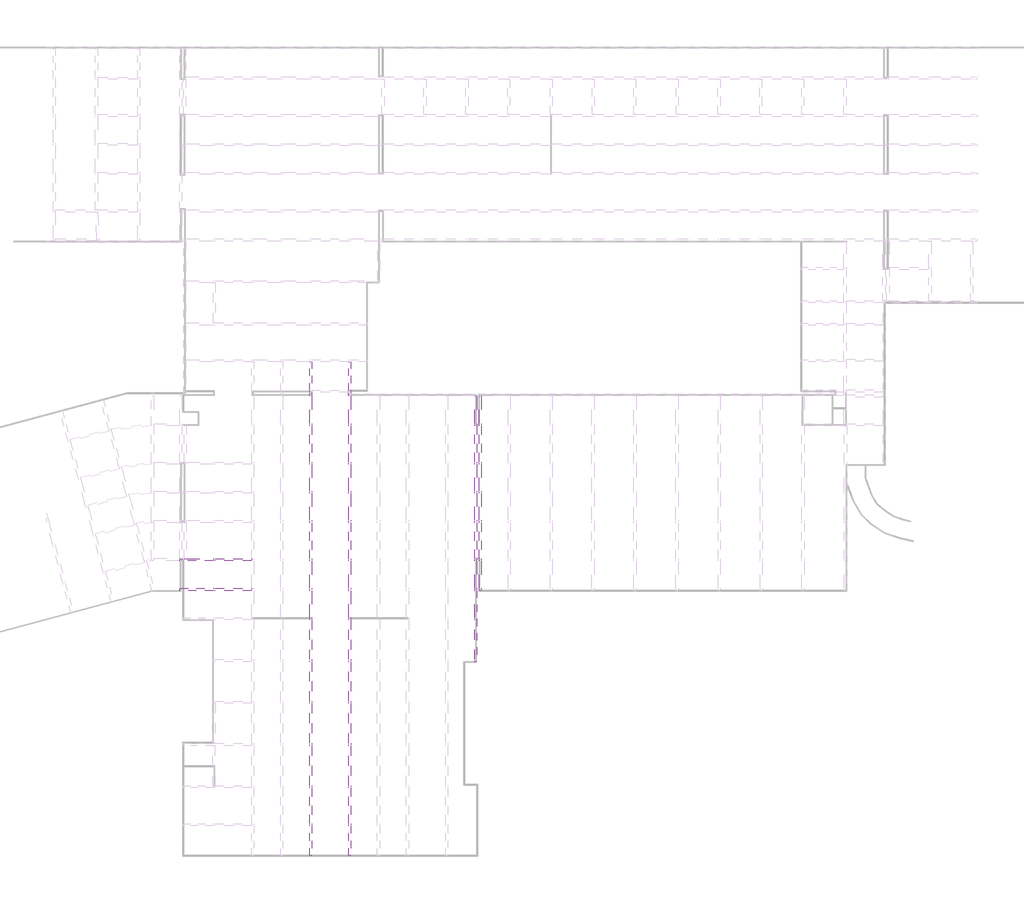
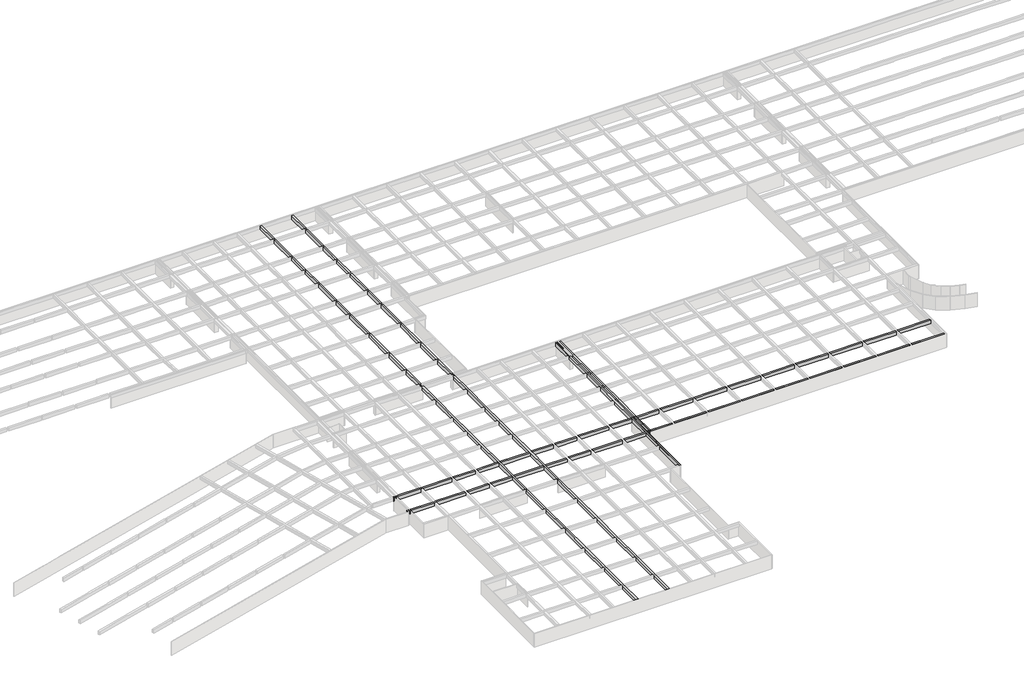
# One storey, part 8 of 14: 6 beams.
"""IFC4 building model written with IfcOpenShell, lengths in millimetres."""

import ifcopenshell
import ifcopenshell.guid

model = None  # the IFC model being written
_history = None  # IfcOwnerHistory: only IFC2X3 demands one
_inside = {}  # id of a spatial element -> (the spatial element, [elements in it])
_under = {}  # id of a project, library or spatial element -> (it, [spatial elements below it])
_declared = {}  # id of a project -> (the project, [libraries it declares])
_typed = {}  # id of a type object -> (the type object, [elements of that type])
_made_of = {}  # id of a material, layer set ... -> (it, [elements and type objects made of it])


def new_model(schema):
    """Start an empty IFC model of exactly this schema.

    Asked for "IFC4X3", IfcOpenShell would pick the latest addendum, in which some entities
    have other attributes; the version numbers below select the first issue.
    IFC2X3 requires an IfcOwnerHistory on every rooted entity: one is made here for all.
    """
    global model, _history
    if schema == "IFC4X3":
        model = ifcopenshell.file(schema_version=(4, 3, 0, 0))
    else:
        model = ifcopenshell.file(schema=schema)
    _inside.clear()
    _under.clear()
    _declared.clear()
    _typed.clear()
    _made_of.clear()
    _history = None
    if model.schema == "IFC2X3":
        org = make("IfcOrganization", Name="unknown")
        user = make(
            "IfcPersonAndOrganization",
            ThePerson=make("IfcPerson", FamilyName="unknown"),
            TheOrganization=org,
        )
        app = make(
            "IfcApplication",
            ApplicationDeveloper=org,
            Version="unknown",
            ApplicationFullName="unknown",
            ApplicationIdentifier="unknown",
        )
        _history = make(
            "IfcOwnerHistory",
            OwningUser=user,
            OwningApplication=app,
            ChangeAction="ADDED",
            CreationDate=0,
        )
    return model


def make(cls, **values):
    """One entity of the class cls with the attributes given. An attribute that is None is left unset."""
    return model.create_entity(
        cls, **{name: value for name, value in values.items() if value is not None}
    )


def rooted(cls, **values):
    """An entity with a GlobalId (a new one), such as an element, a storey or a relation."""
    return make(cls, GlobalId=ifcopenshell.guid.new(), OwnerHistory=_history, **values)


def si_unit(unit_type, name, prefix=None):
    """IfcSIUnit, for example si_unit("LENGTHUNIT", "METRE", prefix="MILLI")."""
    return make("IfcSIUnit", UnitType=unit_type, Prefix=prefix, Name=name)


def assignment(units):
    """IfcUnitAssignment: the units of a project."""
    return None if units is None else make("IfcUnitAssignment", Units=units)


def point(xyz):
    """IfcCartesianPoint."""
    return None if xyz is None else make("IfcCartesianPoint", Coordinates=xyz)


def direction(xyz):
    """IfcDirection."""
    return None if xyz is None else make("IfcDirection", DirectionRatios=xyz)


def frame(location, z_axis=None, x_axis=None):
    """IfcAxis2Placement3D, a coordinate frame: its origin and axes. An axis left out is left unset."""
    return make(
        "IfcAxis2Placement3D",
        Location=point(location),
        Axis=direction(z_axis),
        RefDirection=direction(x_axis),
    )


def origin():
    """The frame at (0, 0, 0) with its axes left unset."""
    return frame((0.0, 0.0, 0.0))


def place(relative_to, where):
    """IfcLocalPlacement: puts the frame where relative to a parent placement (None: the world)."""
    return make(
        "IfcLocalPlacement", PlacementRelTo=relative_to, RelativePlacement=where
    )


def context(
    kind, dimensions, precision=None, world=None, true_north=None, identifier=None
):
    """IfcGeometricRepresentationContext, for example the 3D "Model" context."""
    return make(
        "IfcGeometricRepresentationContext",
        ContextIdentifier=identifier,
        ContextType=kind,
        CoordinateSpaceDimension=dimensions,
        Precision=precision,
        WorldCoordinateSystem=world,
        TrueNorth=true_north,
    )


def project(units=None, contexts=None):
    """IfcProject with its units and contexts."""
    return rooted(
        "IfcProject",
        Name="project",
        RepresentationContexts=contexts,
        UnitsInContext=assignment(units),
    )


def spatial(cls, under=None, at=None, **own):
    """A site, building, storey or space (cls), placed at a placement, below another one or the project."""
    s = rooted(cls, ObjectPlacement=at, **own)
    if under is not None:
        _under.setdefault(under.id(), (under, []))[1].append(s)
    return s


def faces_of(points, faces, orient=None, outer=None):
    """IfcFace entities. A face is a list of loops; a loop is a list of indices into points, from 0.

    orient and outer hold one flag for each loop. By default every Orientation is true, the
    first loop of a face is its IfcFaceOuterBound and the others are IfcFaceBound.
    """
    made = []
    for i, loops in enumerate(faces):
        bounds = []
        for j, loop in enumerate(loops):
            is_outer = j == 0 if outer is None else outer[i][j]
            bounds.append(
                make(
                    "IfcFaceOuterBound" if is_outer else "IfcFaceBound",
                    Bound=make("IfcPolyLoop", Polygon=[points[k] for k in loop]),
                    Orientation=True if orient is None else orient[i][j],
                )
            )
        made.append(make("IfcFace", Bounds=bounds))
    return made


def faceted_brep(points, faces, orient=None, outer=None, voids=None):
    """IfcFacetedBrep: a solid bounded by flat faces; with voids (closed shells), ...WithVoids."""
    shared = [point(p) for p in points]
    hull = make("IfcClosedShell", CfsFaces=faces_of(shared, faces, orient, outer))
    if voids is None:
        return make("IfcFacetedBrep", Outer=hull)
    return make(
        "IfcFacetedBrepWithVoids",
        Outer=hull,
        Voids=[
            make(cls, CfsFaces=faces_of(shared, fs, o, b)) for cls, fs, o, b in voids
        ],
    )


def shape(context_of_items, identifier, shape_type, items):
    """IfcShapeRepresentation: the items that make up one representation, for example the "Body"."""
    return make(
        "IfcShapeRepresentation",
        ContextOfItems=context_of_items,
        RepresentationIdentifier=identifier,
        RepresentationType=shape_type,
        Items=items,
    )


def made_of(thing, what):
    """Note that an element or type object is made of a material, layer set ...; save() writes the relation."""
    if what is not None:
        _made_of.setdefault(what.id(), (what, []))[1].append(thing)
    return thing


def element(
    cls,
    number,
    at=None,
    inside=None,
    cuts=None,
    type_object=None,
    material=None,
    context=None,
    identifier="Body",
    shape_type=None,
    held_by="IfcProductDefinitionShape",
    body=None,
    shapes=None,
    **own,
):
    """One element of the class cls, such as IfcWall. Its Tag is "e" and its number.

    at: its placement. inside: the storey or other place that contains it. cuts: it is an
    opening in that element (IfcRelVoidsElement). A single representation is given by context,
    identifier, shape_type and body (its items); several are given by shapes. held_by: the class
    of the entity that holds the representations. save() writes the other relations.
    """
    e = rooted(cls, Tag="e%d" % number, ObjectPlacement=at, **own)
    if body is not None:
        shapes = [shape(context, identifier, shape_type, body)]
    if shapes is not None:
        e.Representation = make(held_by, Representations=shapes)
    if inside is not None:
        _inside.setdefault(inside.id(), (inside, []))[1].append(e)
    if cuts is not None:
        rooted(
            "IfcRelVoidsElement", RelatingBuildingElement=cuts, RelatedOpeningElement=e
        )
    if type_object is not None:
        _typed.setdefault(type_object.id(), (type_object, []))[1].append(e)
    return made_of(e, material)


def aggregate(whole, parts):
    """IfcRelAggregates: a whole, such as a stair, and the parts it consists of."""
    return rooted("IfcRelAggregates", RelatingObject=whole, RelatedObjects=parts)


def save(model, path):
    """Write the relations noted so far, then the file.

    IfcRelAggregates (storeys below a building ...), IfcRelContainedInSpatialStructure (elements
    in a storey), IfcRelDefinesByType, IfcRelAssociatesMaterial and IfcRelDeclares: one each for
    every whole, place, type object, material and project.
    """
    for whole, parts in _under.values():
        aggregate(whole, parts)
    for where, things in _inside.values():
        rooted(
            "IfcRelContainedInSpatialStructure",
            RelatedElements=things,
            RelatingStructure=where,
        )
    for kind, things in _typed.values():
        rooted("IfcRelDefinesByType", RelatedObjects=things, RelatingType=kind)
    for what, things in _made_of.values():
        rooted("IfcRelAssociatesMaterial", RelatedObjects=things, RelatingMaterial=what)
    for by, libraries in _declared.values():
        rooted("IfcRelDeclares", RelatingContext=by, RelatedDefinitions=libraries)
    model.write(path)


model = new_model("IFC4")

# Units and contexts
model_context = context("Model", 3, world=origin())
ifc_project = project(units=[si_unit("LENGTHUNIT", "METRE", prefix="MILLI")], contexts=[model_context])

# Site, building, storey
site = spatial("IfcSite", under=ifc_project)
building = spatial("IfcBuilding", under=site)
storey = spatial("IfcBuildingStorey", under=building, Name="户型图", Elevation=0.0)

# Beams
placement = place(None, origin())
element("IfcBeam", 1, ObjectType="混凝土 - 矩形梁 : KL_beam", at=placement, inside=storey, context=model_context, shape_type="Brep", body=[
    faceted_brep([(37081.5607309, -267473.0312098, 3300.0), (36681.5607309, -267473.0312098, 3300.0), (36681.5607309, -267473.0312098, 2500.0), (37081.5607309, -267473.0312098, 2500.0), (37081.5607309, -261891.8929199, 3300.0), (37081.5607309, -261491.8929199, 3300.0), (37081.5607309, -254823.1116625, 3300.0), (37081.5607309, -254423.1116625, 3300.0), (37081.5607309, -247008.950757, 3300.0), (37081.5607309, -246608.950757, 3300.0), (37081.5607309, -239178.950757, 3300.0), (37081.5607309, -238778.950757, 3300.0), (37081.5607309, -231409.1116625, 3300.0), (37081.5607309, -231009.1116625, 3300.0), (37081.5607309, -223621.814057, 3300.0), (37081.5607309, -223221.814057, 3300.0), (37081.5607309, -218208.950757, 3300.0), (37081.5607309, -217808.950757, 3300.0), (37081.5607309, -212708.950757, 3300.0), (37081.5607309, -212308.950757, 3300.0), (37081.5607309, -205576.1028577, 3300.0), (37081.5607309, -205176.1028577, 3300.0), (37081.5607309, -200154.952508, 3300.0), (37081.5607309, -199754.952508, 3300.0), (37081.5607309, -194741.3993539, 3300.0), (37081.5607309, -194341.3993539, 3300.0), (37081.5607309, -187598.950757, 3300.0), (37081.5607309, -187198.950757, 3300.0), (37081.5607309, -182068.950757, 3300.0), (37081.5607309, -181668.950757, 3300.0), (37081.5607309, -181394.9655707, 3300.0), (37081.5607309, -180994.9655707, 3300.0), (37081.5607309, -175717.1358924, 3300.0), (36681.5607309, -175717.1358924, 3300.0), (36681.5607309, -180994.9655707, 3300.0), (36681.5607309, -181394.9655707, 3300.0), (36681.5607309, -181668.950757, 3300.0), (36681.5607309, -182068.950757, 3300.0), (36681.5607309, -187198.950757, 3300.0), (36681.5607309, -187598.950757, 3300.0), (36681.5607309, -194341.3993539, 3300.0), (36681.5607309, -194741.3993539, 3300.0), (36681.5607309, -199754.952508, 3300.0), (36681.5607309, -200154.952508, 3300.0), (36681.5607309, -205176.1028577, 3300.0), (36681.5607309, -205576.1028577, 3300.0), (36681.5607309, -212308.950757, 3300.0), (36681.5607309, -212708.950757, 3300.0), (36681.5607309, -217808.950757, 3300.0), (36681.5607309, -218208.950757, 3300.0), (36681.5607309, -223221.814057, 3300.0), (36681.5607309, -223621.814057, 3300.0), (36681.5607309, -231009.1116625, 3300.0), (36681.5607309, -231409.1116625, 3300.0), (36681.5607309, -238778.950757, 3300.0), (36681.5607309, -239178.950757, 3300.0), (36681.5607309, -246608.950757, 3300.0), (36681.5607309, -247008.950757, 3300.0), (36681.5607309, -254423.1116625, 3300.0), (36681.5607309, -254823.1116625, 3300.0), (36681.5607309, -261491.8929199, 3300.0), (36681.5607309, -261891.8929199, 3300.0), (36681.5607309, -175717.1358924, 2500.0), (36681.5607309, -180994.9655707, 2500.0), (36681.5607309, -181394.9655707, 2500.0), (36681.5607309, -181668.950757, 2500.0), (36681.5607309, -182068.950757, 2500.0), (36681.5607309, -187198.950757, 2500.0), (36681.5607309, -187598.950757, 2500.0), (36681.5607309, -194341.3993539, 2500.0), (36681.5607309, -194741.3993539, 2500.0), (36681.5607309, -199754.952508, 2500.0), (36681.5607309, -200154.952508, 2500.0), (36681.5607309, -205176.1028577, 2500.0), (36681.5607309, -205576.1028577, 2500.0), (36681.5607309, -212308.950757, 2500.0), (36681.5607309, -212708.950757, 2500.0), (36681.5607309, -217808.950757, 2500.0), (36681.5607309, -218208.950757, 2500.0), (36681.5607309, -223221.814057, 2500.0), (36681.5607309, -223621.814057, 2500.0), (36681.5607309, -231009.1116625, 2500.0), (36681.5607309, -231409.1116625, 2500.0), (36681.5607309, -238778.950757, 2500.0), (36681.5607309, -239178.950757, 2500.0), (36681.5607309, -246608.950757, 2500.0), (36681.5607309, -247008.950757, 2500.0), (36681.5607309, -254423.1116625, 2500.0), (36681.5607309, -254823.1116625, 2500.0), (36681.5607309, -261491.8929199, 2500.0), (36681.5607309, -261891.8929199, 2500.0), (37081.5607309, -175717.1358924, 2500.0), (37081.5607309, -180994.9655707, 2500.0), (37081.5607309, -181394.9655707, 2500.0), (37081.5607309, -181668.950757, 2500.0), (37081.5607309, -182068.950757, 2500.0), (37081.5607309, -187198.950757, 2500.0), (37081.5607309, -187598.950757, 2500.0), (37081.5607309, -194341.3993539, 2500.0), (37081.5607309, -194741.3993539, 2500.0), (37081.5607309, -199754.952508, 2500.0), (37081.5607309, -200154.952508, 2500.0), (37081.5607309, -205176.1028577, 2500.0), (37081.5607309, -205576.1028577, 2500.0), (37081.5607309, -212308.950757, 2500.0), (37081.5607309, -212708.950757, 2500.0), (37081.5607309, -217808.950757, 2500.0), (37081.5607309, -218208.950757, 2500.0), (37081.5607309, -223221.814057, 2500.0), (37081.5607309, -223621.814057, 2500.0), (37081.5607309, -231009.1116625, 2500.0), (37081.5607309, -231409.1116625, 2500.0), (37081.5607309, -238778.950757, 2500.0), (37081.5607309, -239178.950757, 2500.0), (37081.5607309, -246608.950757, 2500.0), (37081.5607309, -247008.950757, 2500.0), (37081.5607309, -254423.1116625, 2500.0), (37081.5607309, -254823.1116625, 2500.0), (37081.5607309, -261491.8929199, 2500.0), (37081.5607309, -261891.8929199, 2500.0)], [[[0, 1, 2, 3]], [[1, 0, 4, 5, 6, 7, 8, 9, 10, 11, 12, 13, 14, 15, 16, 17, 18, 19, 20, 21, 22, 23, 24, 25, 26, 27, 28, 29, 30, 31, 32, 33, 34, 35, 36, 37, 38, 39, 40, 41, 42, 43, 44, 45, 46, 47, 48, 49, 50, 51, 52, 53, 54, 55, 56, 57, 58, 59, 60, 61]], [[2, 1, 61, 60, 59, 58, 57, 56, 55, 54, 53, 52, 51, 50, 49, 48, 47, 46, 45, 44, 43, 42, 41, 40, 39, 38, 37, 36, 35, 34, 33, 62, 63, 64, 65, 66, 67, 68, 69, 70, 71, 72, 73, 74, 75, 76, 77, 78, 79, 80, 81, 82, 83, 84, 85, 86, 87, 88, 89, 90]], [[3, 2, 90, 89, 88, 87, 86, 85, 84, 83, 82, 81, 80, 79, 78, 77, 76, 75, 74, 73, 72, 71, 70, 69, 68, 67, 66, 65, 64, 63, 62, 91, 92, 93, 94, 95, 96, 97, 98, 99, 100, 101, 102, 103, 104, 105, 106, 107, 108, 109, 110, 111, 112, 113, 114, 115, 116, 117, 118, 119]], [[0, 3, 119, 118, 117, 116, 115, 114, 113, 112, 111, 110, 109, 108, 107, 106, 105, 104, 103, 102, 101, 100, 99, 98, 97, 96, 95, 94, 93, 92, 91, 32, 31, 30, 29, 28, 27, 26, 25, 24, 23, 22, 21, 20, 19, 18, 17, 16, 15, 14, 13, 12, 11, 10, 9, 8, 7, 6, 5, 4]], [[33, 32, 91, 62]]]),
    faceted_brep([(36681.5607309, -123197.8127788, 3300.0), (37081.5607309, -123197.8127788, 3300.0), (37081.5607309, -123197.8127788, 2500.0), (36681.5607309, -123197.8127788, 2500.0), (37081.5607309, -129780.0179086, 3300.0), (36681.5607309, -129780.0179086, 3300.0), (36681.5607309, -129780.0179086, 2500.0), (37081.5607309, -129780.0179086, 2500.0)], [[[0, 1, 2, 3]], [[4, 5, 6, 7]], [[1, 0, 5, 4]], [[0, 3, 6, 5]], [[3, 2, 7, 6]], [[2, 1, 4, 7]]]),
    faceted_brep([(37081.5607309, -122797.8127788, 3300.0), (36681.5607309, -122797.8127788, 3300.0), (36681.5607309, -122797.8127788, 2500.0), (37081.5607309, -122797.8127788, 2500.0), (37081.5607309, -117558.950757, 3300.0), (36681.5607309, -117558.950757, 3300.0), (36681.5607309, -117558.950757, 2500.0), (37081.5607309, -117558.950757, 2500.0)], [[[0, 1, 2, 3]], [[1, 0, 4, 5]], [[2, 1, 5, 6]], [[3, 2, 6, 7]], [[0, 3, 7, 4]], [[5, 4, 7, 6]]]),
    faceted_brep([(36681.5607309, -130180.0179086, 3300.0), (37081.5607309, -130180.0179086, 3300.0), (37081.5607309, -130180.0179086, 2500.0), (36681.5607309, -130180.0179086, 2500.0), (37081.5607309, -135180.0179086, 3300.0), (36681.5607309, -135180.0179086, 3300.0), (36681.5607309, -135180.0179086, 2500.0), (37081.5607309, -135180.0179086, 2500.0)], [[[0, 1, 2, 3]], [[4, 5, 6, 7]], [[1, 0, 5, 4]], [[0, 3, 6, 5]], [[3, 2, 7, 6]], [[2, 1, 4, 7]]]),
    faceted_brep([(36681.5607309, -135580.0179086, 3300.0), (37081.5607309, -135580.0179086, 3300.0), (37081.5607309, -135580.0179086, 2500.0), (36681.5607309, -135580.0179086, 2500.0), (37081.5607309, -140520.0179086, 3300.0), (36681.5607309, -140520.0179086, 3300.0), (36681.5607309, -140520.0179086, 2500.0), (37081.5607309, -140520.0179086, 2500.0)], [[[0, 1, 2, 3]], [[4, 5, 6, 7]], [[1, 0, 5, 4]], [[0, 3, 6, 5]], [[3, 2, 7, 6]], [[2, 1, 4, 7]]]),
    faceted_brep([(36681.5607309, -140920.0179086, 3300.0), (37081.5607309, -140920.0179086, 3300.0), (37081.5607309, -140920.0179086, 2500.0), (36681.5607309, -140920.0179086, 2500.0), (37081.5607309, -147499.284307, 3300.0), (36681.5607309, -147499.284307, 3300.0), (36681.5607309, -147499.284307, 2500.0), (37081.5607309, -147499.284307, 2500.0)], [[[0, 1, 2, 3]], [[4, 5, 6, 7]], [[1, 0, 5, 4]], [[0, 3, 6, 5]], [[3, 2, 7, 6]], [[2, 1, 4, 7]]]),
    faceted_brep([(36681.5607309, -147899.284307, 3300.0), (37081.5607309, -147899.284307, 3300.0), (37081.5607309, -147899.284307, 2500.0), (36681.5607309, -147899.284307, 2500.0), (37081.5607309, -152899.284307, 3300.0), (36681.5607309, -152899.284307, 3300.0), (36681.5607309, -152899.284307, 2500.0), (37081.5607309, -152899.284307, 2500.0)], [[[0, 1, 2, 3]], [[4, 5, 6, 7]], [[1, 0, 5, 4]], [[0, 3, 6, 5]], [[3, 2, 7, 6]], [[2, 1, 4, 7]]]),
    faceted_brep([(36681.5607309, -153299.284307, 3300.0), (37081.5607309, -153299.284307, 3300.0), (37081.5607309, -153299.284307, 2500.0), (36681.5607309, -153299.284307, 2500.0), (37081.5607309, -160620.767119, 3300.0), (36681.5607309, -160620.767119, 3300.0), (36681.5607309, -160620.767119, 2500.0), (37081.5607309, -160620.767119, 2500.0)], [[[0, 1, 2, 3]], [[4, 5, 6, 7]], [[1, 0, 5, 4]], [[0, 3, 6, 5]], [[3, 2, 7, 6]], [[2, 1, 4, 7]]]),
    faceted_brep([(36681.5607309, -161020.767119, 3300.0), (37081.5607309, -161020.767119, 3300.0), (37081.5607309, -161020.767119, 2500.0), (36681.5607309, -161020.767119, 2500.0), (37081.5607309, -168501.0793872, 3300.0), (36681.5607309, -168501.0793872, 3300.0), (36681.5607309, -168501.0793872, 2500.0), (37081.5607309, -168501.0793872, 2500.0)], [[[0, 1, 2, 3]], [[4, 5, 6, 7]], [[1, 0, 5, 4]], [[0, 3, 6, 5]], [[3, 2, 7, 6]], [[2, 1, 4, 7]]]),
    faceted_brep([(36681.5607309, -168901.0793872, 3300.0), (37081.5607309, -168901.0793872, 3300.0), (37081.5607309, -168901.0793872, 2500.0), (36681.5607309, -168901.0793872, 2500.0), (37081.5607309, -175317.1358924, 3300.0), (36681.5607309, -175317.1358924, 3300.0), (36681.5607309, -175317.1358924, 2500.0), (37081.5607309, -175317.1358924, 2500.0)], [[[0, 1, 2, 3]], [[4, 5, 6, 7]], [[1, 0, 5, 4]], [[0, 3, 6, 5]], [[3, 2, 7, 6]], [[2, 1, 4, 7]]]),
])
element("IfcBeam", 2, ObjectType="混凝土 - 矩形梁 : KL_beam", at=placement, inside=storey, context=model_context, shape_type="Brep", body=[
    faceted_brep([(43931.9066405, -267473.0312098, 3300.0), (43931.9066405, -267473.0312098, 2500.0), (44331.9066405, -267473.0312098, 2500.0), (44331.9066405, -267473.0312098, 3300.0), (43931.9066405, -175717.1358924, 3300.0), (44331.9066405, -175717.1358924, 3300.0), (44331.9066405, -175717.1358924, 2500.0), (43931.9066405, -175717.1358924, 2500.0), (44331.9066405, -261891.8929199, 3300.0), (44331.9066405, -261491.8929199, 3300.0), (44331.9066405, -254823.1116625, 3300.0), (44331.9066405, -254423.1116625, 3300.0), (44331.9066405, -247008.950757, 3300.0), (44331.9066405, -246608.950757, 3300.0), (44331.9066405, -239178.950757, 3300.0), (44331.9066405, -238778.950757, 3300.0), (44331.9066405, -231409.1116625, 3300.0), (44331.9066405, -231009.1116625, 3300.0), (44331.9066405, -223621.814057, 3300.0), (44331.9066405, -223221.814057, 3300.0), (44331.9066405, -218208.950757, 3300.0), (44331.9066405, -217808.950757, 3300.0), (44331.9066405, -212708.950757, 3300.0), (44331.9066405, -212308.950757, 3300.0), (44331.9066405, -205576.1028577, 3300.0), (44331.9066405, -205176.1028577, 3300.0), (44331.9066405, -200154.952508, 3300.0), (44331.9066405, -199754.952508, 3300.0), (44331.9066405, -194741.3993539, 3300.0), (44331.9066405, -194341.3993539, 3300.0), (44331.9066405, -187598.950757, 3300.0), (44331.9066405, -187198.950757, 3300.0), (44331.9066405, -182068.950757, 3300.0), (44331.9066405, -181668.950757, 3300.0), (44331.9066405, -181394.9655707, 3300.0), (44331.9066405, -180994.9655707, 3300.0), (43931.9066405, -180994.9655707, 3300.0), (43931.9066405, -181394.9655707, 3300.0), (43931.9066405, -181668.950757, 3300.0), (43931.9066405, -182068.950757, 3300.0), (43931.9066405, -187198.950757, 3300.0), (43931.9066405, -187598.950757, 3300.0), (43931.9066405, -194341.3993539, 3300.0), (43931.9066405, -194741.3993539, 3300.0), (43931.9066405, -199754.952508, 3300.0), (43931.9066405, -200154.952508, 3300.0), (43931.9066405, -205176.1028577, 3300.0), (43931.9066405, -205576.1028577, 3300.0), (43931.9066405, -212308.950757, 3300.0), (43931.9066405, -212708.950757, 3300.0), (43931.9066405, -217808.950757, 3300.0), (43931.9066405, -218208.950757, 3300.0), (43931.9066405, -223221.814057, 3300.0), (43931.9066405, -223621.814057, 3300.0), (43931.9066405, -231009.1116625, 3300.0), (43931.9066405, -231409.1116625, 3300.0), (43931.9066405, -238778.950757, 3300.0), (43931.9066405, -239178.950757, 3300.0), (43931.9066405, -246608.950757, 3300.0), (43931.9066405, -247008.950757, 3300.0), (43931.9066405, -254423.1116625, 3300.0), (43931.9066405, -254823.1116625, 3300.0), (43931.9066405, -261491.8929199, 3300.0), (43931.9066405, -261891.8929199, 3300.0), (44331.9066405, -261891.8929199, 2500.0), (44331.9066405, -261491.8929199, 2500.0), (44331.9066405, -254823.1116625, 2500.0), (44331.9066405, -254423.1116625, 2500.0), (44331.9066405, -247008.950757, 2500.0), (44331.9066405, -246608.950757, 2500.0), (44331.9066405, -239178.950757, 2500.0), (44331.9066405, -238778.950757, 2500.0), (44331.9066405, -231409.1116625, 2500.0), (44331.9066405, -231009.1116625, 2500.0), (44331.9066405, -223621.814057, 2500.0), (44331.9066405, -223221.814057, 2500.0), (44331.9066405, -218208.950757, 2500.0), (44331.9066405, -217808.950757, 2500.0), (44331.9066405, -212708.950757, 2500.0), (44331.9066405, -212308.950757, 2500.0), (44331.9066405, -205576.1028577, 2500.0), (44331.9066405, -205176.1028577, 2500.0), (44331.9066405, -200154.952508, 2500.0), (44331.9066405, -199754.952508, 2500.0), (44331.9066405, -194741.3993539, 2500.0), (44331.9066405, -194341.3993539, 2500.0), (44331.9066405, -187598.950757, 2500.0), (44331.9066405, -187198.950757, 2500.0), (44331.9066405, -182068.950757, 2500.0), (44331.9066405, -181668.950757, 2500.0), (44331.9066405, -181394.9655707, 2500.0), (44331.9066405, -180994.9655707, 2500.0), (43931.9066405, -261891.8929199, 2500.0), (43931.9066405, -261491.8929199, 2500.0), (43931.9066405, -254823.1116625, 2500.0), (43931.9066405, -254423.1116625, 2500.0), (43931.9066405, -247008.950757, 2500.0), (43931.9066405, -246608.950757, 2500.0), (43931.9066405, -239178.950757, 2500.0), (43931.9066405, -238778.950757, 2500.0), (43931.9066405, -231409.1116625, 2500.0), (43931.9066405, -231009.1116625, 2500.0), (43931.9066405, -223621.814057, 2500.0), (43931.9066405, -223221.814057, 2500.0), (43931.9066405, -218208.950757, 2500.0), (43931.9066405, -217808.950757, 2500.0), (43931.9066405, -212708.950757, 2500.0), (43931.9066405, -212308.950757, 2500.0), (43931.9066405, -205576.1028577, 2500.0), (43931.9066405, -205176.1028577, 2500.0), (43931.9066405, -200154.952508, 2500.0), (43931.9066405, -199754.952508, 2500.0), (43931.9066405, -194741.3993539, 2500.0), (43931.9066405, -194341.3993539, 2500.0), (43931.9066405, -187598.950757, 2500.0), (43931.9066405, -187198.950757, 2500.0), (43931.9066405, -182068.950757, 2500.0), (43931.9066405, -181668.950757, 2500.0), (43931.9066405, -181394.9655707, 2500.0), (43931.9066405, -180994.9655707, 2500.0)], [[[0, 1, 2, 3]], [[4, 5, 6, 7]], [[0, 3, 8, 9, 10, 11, 12, 13, 14, 15, 16, 17, 18, 19, 20, 21, 22, 23, 24, 25, 26, 27, 28, 29, 30, 31, 32, 33, 34, 35, 5, 4, 36, 37, 38, 39, 40, 41, 42, 43, 44, 45, 46, 47, 48, 49, 50, 51, 52, 53, 54, 55, 56, 57, 58, 59, 60, 61, 62, 63]], [[3, 2, 64, 65, 66, 67, 68, 69, 70, 71, 72, 73, 74, 75, 76, 77, 78, 79, 80, 81, 82, 83, 84, 85, 86, 87, 88, 89, 90, 91, 6, 5, 35, 34, 33, 32, 31, 30, 29, 28, 27, 26, 25, 24, 23, 22, 21, 20, 19, 18, 17, 16, 15, 14, 13, 12, 11, 10, 9, 8]], [[2, 1, 92, 93, 94, 95, 96, 97, 98, 99, 100, 101, 102, 103, 104, 105, 106, 107, 108, 109, 110, 111, 112, 113, 114, 115, 116, 117, 118, 119, 7, 6, 91, 90, 89, 88, 87, 86, 85, 84, 83, 82, 81, 80, 79, 78, 77, 76, 75, 74, 73, 72, 71, 70, 69, 68, 67, 66, 65, 64]], [[1, 0, 63, 62, 61, 60, 59, 58, 57, 56, 55, 54, 53, 52, 51, 50, 49, 48, 47, 46, 45, 44, 43, 42, 41, 40, 39, 38, 37, 36, 4, 7, 119, 118, 117, 116, 115, 114, 113, 112, 111, 110, 109, 108, 107, 106, 105, 104, 103, 102, 101, 100, 99, 98, 97, 96, 95, 94, 93, 92]]]),
    faceted_brep([(43931.9066405, -122797.8127788, 3300.0), (44331.9066405, -122797.8127788, 3300.0), (44331.9066405, -117558.950757, 3300.0), (43931.9066405, -117558.950757, 3300.0), (44331.9066405, -122797.8127788, 2500.0), (44331.9066405, -117558.950757, 2500.0), (43931.9066405, -122797.8127788, 2500.0), (43931.9066405, -117558.950757, 2500.0)], [[[0, 1, 2, 3]], [[1, 4, 5, 2]], [[4, 6, 7, 5]], [[6, 0, 3, 7]], [[1, 0, 6, 4]], [[3, 2, 5, 7]]]),
    faceted_brep([(43931.9066405, -123197.8127788, 3300.0), (44331.9066405, -123197.8127788, 3300.0), (44331.9066405, -123197.8127788, 2500.0), (43931.9066405, -123197.8127788, 2500.0), (43931.9066405, -129780.0179086, 3300.0), (44331.9066405, -129780.0179086, 3300.0), (44331.9066405, -129780.0179086, 2500.0), (43931.9066405, -129780.0179086, 2500.0)], [[[0, 1, 2, 3]], [[1, 0, 4, 5]], [[2, 1, 5, 6]], [[3, 2, 6, 7]], [[0, 3, 7, 4]], [[5, 4, 7, 6]]]),
    faceted_brep([(43931.9066405, -130180.0179086, 3300.0), (44331.9066405, -130180.0179086, 3300.0), (44331.9066405, -130180.0179086, 2500.0), (43931.9066405, -130180.0179086, 2500.0), (43931.9066405, -135180.0179086, 3300.0), (44331.9066405, -135180.0179086, 3300.0), (44331.9066405, -135180.0179086, 2500.0), (43931.9066405, -135180.0179086, 2500.0)], [[[0, 1, 2, 3]], [[1, 0, 4, 5]], [[2, 1, 5, 6]], [[3, 2, 6, 7]], [[0, 3, 7, 4]], [[5, 4, 7, 6]]]),
    faceted_brep([(43931.9066405, -135580.0179086, 3300.0), (44331.9066405, -135580.0179086, 3300.0), (44331.9066405, -135580.0179086, 2500.0), (43931.9066405, -135580.0179086, 2500.0), (43931.9066405, -140520.0179086, 3300.0), (44331.9066405, -140520.0179086, 3300.0), (44331.9066405, -140520.0179086, 2500.0), (43931.9066405, -140520.0179086, 2500.0)], [[[0, 1, 2, 3]], [[1, 0, 4, 5]], [[2, 1, 5, 6]], [[3, 2, 6, 7]], [[0, 3, 7, 4]], [[5, 4, 7, 6]]]),
    faceted_brep([(43931.9066405, -140920.0179086, 3300.0), (44331.9066405, -140920.0179086, 3300.0), (44331.9066405, -140920.0179086, 2500.0), (43931.9066405, -140920.0179086, 2500.0), (43931.9066405, -147499.284307, 3300.0), (44331.9066405, -147499.284307, 3300.0), (44331.9066405, -147499.284307, 2500.0), (43931.9066405, -147499.284307, 2500.0)], [[[0, 1, 2, 3]], [[1, 0, 4, 5]], [[2, 1, 5, 6]], [[3, 2, 6, 7]], [[0, 3, 7, 4]], [[5, 4, 7, 6]]]),
    faceted_brep([(43931.9066405, -147899.284307, 3300.0), (44331.9066405, -147899.284307, 3300.0), (44331.9066405, -147899.284307, 2500.0), (43931.9066405, -147899.284307, 2500.0), (43931.9066405, -152899.284307, 3300.0), (44331.9066405, -152899.284307, 3300.0), (44331.9066405, -152899.284307, 2500.0), (43931.9066405, -152899.284307, 2500.0)], [[[0, 1, 2, 3]], [[1, 0, 4, 5]], [[2, 1, 5, 6]], [[3, 2, 6, 7]], [[0, 3, 7, 4]], [[5, 4, 7, 6]]]),
    faceted_brep([(43931.9066405, -153299.284307, 3300.0), (44331.9066405, -153299.284307, 3300.0), (44331.9066405, -153299.284307, 2500.0), (43931.9066405, -153299.284307, 2500.0), (43931.9066405, -160620.767119, 3300.0), (44331.9066405, -160620.767119, 3300.0), (44331.9066405, -160620.767119, 2500.0), (43931.9066405, -160620.767119, 2500.0)], [[[0, 1, 2, 3]], [[1, 0, 4, 5]], [[2, 1, 5, 6]], [[3, 2, 6, 7]], [[0, 3, 7, 4]], [[5, 4, 7, 6]]]),
    faceted_brep([(43931.9066405, -161020.767119, 3300.0), (44331.9066405, -161020.767119, 3300.0), (44331.9066405, -161020.767119, 2500.0), (43931.9066405, -161020.767119, 2500.0), (43931.9066405, -168501.0793872, 3300.0), (44331.9066405, -168501.0793872, 3300.0), (44331.9066405, -168501.0793872, 2500.0), (43931.9066405, -168501.0793872, 2500.0)], [[[0, 1, 2, 3]], [[1, 0, 4, 5]], [[2, 1, 5, 6]], [[3, 2, 6, 7]], [[0, 3, 7, 4]], [[5, 4, 7, 6]]]),
    faceted_brep([(43931.9066405, -168901.0793872, 3300.0), (44331.9066405, -168901.0793872, 3300.0), (44331.9066405, -168901.0793872, 2500.0), (43931.9066405, -168901.0793872, 2500.0), (43931.9066405, -175317.1358924, 3300.0), (44331.9066405, -175317.1358924, 3300.0), (44331.9066405, -175317.1358924, 2500.0), (43931.9066405, -175317.1358924, 2500.0)], [[[0, 1, 2, 3]], [[1, 0, 4, 5]], [[2, 1, 5, 6]], [[3, 2, 6, 7]], [[0, 3, 7, 4]], [[5, 4, 7, 6]]]),
])
element("IfcBeam", 3, ObjectType="混凝土 - 矩形梁 : KL_beam", at=placement, inside=storey, context=model_context, shape_type="Brep", body=[
    faceted_brep([(67367.2949044, -231409.1116625, 3300.0), (67767.2949044, -231409.1116625, 3300.0), (67767.2949044, -218208.950757, 3300.0), (67767.2949044, -217808.950757, 3300.0), (67767.2949044, -212708.950757, 3300.0), (67767.2949044, -212308.950757, 3300.0), (67767.2949044, -205576.1028577, 3300.0), (67767.2949044, -205176.1028577, 3300.0), (67767.2949044, -200154.952508, 3300.0), (67767.2949044, -199754.952508, 3300.0), (67767.2949044, -194741.3993539, 3300.0), (67767.2949044, -194341.3993539, 3300.0), (67767.2949044, -187598.950757, 3300.0), (67767.2949044, -187198.950757, 3300.0), (67767.2949044, -182068.950757, 3300.0), (67367.2949044, -182068.950757, 3300.0), (67367.2949044, -187198.950757, 3300.0), (67367.2949044, -187598.950757, 3300.0), (67367.2949044, -194341.3993539, 3300.0), (67367.2949044, -194741.3993539, 3300.0), (67367.2949044, -199754.952508, 3300.0), (67367.2949044, -200154.952508, 3300.0), (67367.2949044, -205176.1028577, 3300.0), (67367.2949044, -205576.1028577, 3300.0), (67367.2949044, -212308.950757, 3300.0), (67367.2949044, -212708.950757, 3300.0), (67367.2949044, -217808.950757, 3300.0), (67367.2949044, -218208.950757, 3300.0), (67367.2949044, -223221.814057, 3300.0), (67367.2949044, -223621.814057, 3300.0), (67367.2949044, -231009.1116625, 3300.0), (67367.2949044, -231409.1116625, 2500.0), (67367.2949044, -182068.950757, 2500.0), (67367.2949044, -187198.950757, 2500.0), (67367.2949044, -187598.950757, 2500.0), (67367.2949044, -194341.3993539, 2500.0), (67367.2949044, -194741.3993539, 2500.0), (67367.2949044, -199754.952508, 2500.0), (67367.2949044, -200154.952508, 2500.0), (67367.2949044, -205176.1028577, 2500.0), (67367.2949044, -205576.1028577, 2500.0), (67367.2949044, -212308.950757, 2500.0), (67367.2949044, -212708.950757, 2500.0), (67367.2949044, -217808.950757, 2500.0), (67367.2949044, -218208.950757, 2500.0), (67367.2949044, -223221.814057, 2500.0), (67367.2949044, -223621.814057, 2500.0), (67367.2949044, -231009.1116625, 2500.0), (67767.2949044, -231409.1116625, 2500.0), (67767.2949044, -182068.950757, 2500.0), (67767.2949044, -187198.950757, 2500.0), (67767.2949044, -187598.950757, 2500.0), (67767.2949044, -194341.3993539, 2500.0), (67767.2949044, -194741.3993539, 2500.0), (67767.2949044, -199754.952508, 2500.0), (67767.2949044, -200154.952508, 2500.0), (67767.2949044, -205176.1028577, 2500.0), (67767.2949044, -205576.1028577, 2500.0), (67767.2949044, -212308.950757, 2500.0), (67767.2949044, -212708.950757, 2500.0), (67767.2949044, -217808.950757, 2500.0), (67767.2949044, -218208.950757, 2500.0)], [[[0, 1, 2, 3, 4, 5, 6, 7, 8, 9, 10, 11, 12, 13, 14, 15, 16, 17, 18, 19, 20, 21, 22, 23, 24, 25, 26, 27, 28, 29, 30]], [[31, 0, 30, 29, 28, 27, 26, 25, 24, 23, 22, 21, 20, 19, 18, 17, 16, 15, 32, 33, 34, 35, 36, 37, 38, 39, 40, 41, 42, 43, 44, 45, 46, 47]], [[48, 31, 47, 46, 45, 44, 43, 42, 41, 40, 39, 38, 37, 36, 35, 34, 33, 32, 49, 50, 51, 52, 53, 54, 55, 56, 57, 58, 59, 60, 61]], [[1, 48, 61, 60, 59, 58, 57, 56, 55, 54, 53, 52, 51, 50, 49, 14, 13, 12, 11, 10, 9, 8, 7, 6, 5, 4, 3, 2]], [[15, 14, 49, 32]], [[1, 0, 31, 48]]]),
])
element("IfcBeam", 4, ObjectType="混凝土 - 矩形梁 : KL_beam", at=placement, inside=storey, context=model_context, shape_type="Brep", body=[
    faceted_brep([(68177.2949044, -218258.950757, 3300.0), (68177.2949044, -218258.950757, 2500.0), (68577.2949044, -218258.950757, 2500.0), (68577.2949044, -218258.950757, 3300.0), (68577.2949044, -218208.950757, 3300.0), (68577.2949044, -217808.950757, 3300.0), (68577.2949044, -212708.950757, 3300.0), (68577.2949044, -212308.950757, 3300.0), (68577.2949044, -205576.1028577, 3300.0), (68577.2949044, -205176.1028577, 3300.0), (68577.2949044, -200154.952508, 3300.0), (68577.2949044, -199754.952508, 3300.0), (68577.2949044, -194741.3993539, 3300.0), (68577.2949044, -194341.3993539, 3300.0), (68577.2949044, -187598.950757, 3300.0), (68577.2949044, -187198.950757, 3300.0), (68577.2949044, -182068.950757, 3300.0), (68177.2949044, -182068.950757, 3300.0), (68177.2949044, -187198.950757, 3300.0), (68177.2949044, -187598.950757, 3300.0), (68177.2949044, -194341.3993539, 3300.0), (68177.2949044, -194741.3993539, 3300.0), (68177.2949044, -199754.952508, 3300.0), (68177.2949044, -200154.952508, 3300.0), (68177.2949044, -205176.1028577, 3300.0), (68177.2949044, -205576.1028577, 3300.0), (68177.2949044, -212308.950757, 3300.0), (68177.2949044, -212708.950757, 3300.0), (68177.2949044, -217808.950757, 3300.0), (68177.2949044, -218208.950757, 3300.0), (68577.2949044, -218208.950757, 2500.0), (68577.2949044, -217808.950757, 2500.0), (68577.2949044, -212708.950757, 2500.0), (68577.2949044, -212308.950757, 2500.0), (68577.2949044, -205576.1028577, 2500.0), (68577.2949044, -205176.1028577, 2500.0), (68577.2949044, -200154.952508, 2500.0), (68577.2949044, -199754.952508, 2500.0), (68577.2949044, -194741.3993539, 2500.0), (68577.2949044, -194341.3993539, 2500.0), (68577.2949044, -187598.950757, 2500.0), (68577.2949044, -187198.950757, 2500.0), (68577.2949044, -182068.950757, 2500.0), (68177.2949044, -218208.950757, 2500.0), (68177.2949044, -217808.950757, 2500.0), (68177.2949044, -212708.950757, 2500.0), (68177.2949044, -212308.950757, 2500.0), (68177.2949044, -205576.1028577, 2500.0), (68177.2949044, -205176.1028577, 2500.0), (68177.2949044, -200154.952508, 2500.0), (68177.2949044, -199754.952508, 2500.0), (68177.2949044, -194741.3993539, 2500.0), (68177.2949044, -194341.3993539, 2500.0), (68177.2949044, -187598.950757, 2500.0), (68177.2949044, -187198.950757, 2500.0), (68177.2949044, -182068.950757, 2500.0)], [[[0, 1, 2, 3]], [[0, 3, 4, 5, 6, 7, 8, 9, 10, 11, 12, 13, 14, 15, 16, 17, 18, 19, 20, 21, 22, 23, 24, 25, 26, 27, 28, 29]], [[3, 2, 30, 31, 32, 33, 34, 35, 36, 37, 38, 39, 40, 41, 42, 16, 15, 14, 13, 12, 11, 10, 9, 8, 7, 6, 5, 4]], [[2, 1, 43, 44, 45, 46, 47, 48, 49, 50, 51, 52, 53, 54, 55, 42, 41, 40, 39, 38, 37, 36, 35, 34, 33, 32, 31, 30]], [[1, 0, 29, 28, 27, 26, 25, 24, 23, 22, 21, 20, 19, 18, 17, 55, 54, 53, 52, 51, 50, 49, 48, 47, 46, 45, 44, 43]], [[17, 16, 42, 55]]]),
])
element("IfcBeam", 5, ObjectType="混凝土 - 矩形梁 : KL_beam", at=placement, inside=storey, context=model_context, shape_type="Brep", body=[
    faceted_brep([(136047.2949044, -212708.950757, 3300.0), (136047.2949044, -212308.950757, 3300.0), (128549.172254, -212308.950757, 3300.0), (128549.172254, -212708.950757, 3300.0), (136047.2949044, -212308.950757, 2500.0), (128549.172254, -212308.950757, 2500.0), (136047.2949044, -212708.950757, 2500.0), (128549.172254, -212708.950757, 2500.0)], [[[0, 1, 2, 3]], [[1, 4, 5, 2]], [[4, 6, 7, 5]], [[6, 0, 3, 7]], [[1, 0, 6, 4]], [[3, 2, 5, 7]]]),
    faceted_brep([(25921.5607309, -212308.950757, 3300.0), (25921.5607309, -212708.950757, 3300.0), (25921.5607309, -212708.950757, 2500.0), (25921.5607309, -212308.950757, 2500.0), (19160.0865653, -212308.950757, 3300.0), (18760.0865653, -212308.950757, 3300.0), (13777.4621399, -212308.950757, 3300.0), (13377.4621399, -212308.950757, 3300.0), (12933.1378826, -212308.950757, 3300.0), (12533.1378826, -212308.950757, 3300.0), (12533.1378826, -212638.9019002, 3300.0), (12533.1378826, -212708.950757, 3300.0), (18760.0865653, -212708.950757, 3300.0), (19160.0865653, -212708.950757, 3300.0), (19160.0865653, -212308.950757, 2500.0), (18760.0865653, -212308.950757, 2500.0), (13777.4621399, -212308.950757, 2500.0), (13377.4621399, -212308.950757, 2500.0), (12933.1378826, -212308.950757, 2500.0), (12533.1378826, -212308.950757, 2500.0), (19160.0865653, -212708.950757, 2500.0), (18760.0865653, -212708.950757, 2500.0), (12533.1378826, -212708.950757, 2500.0), (12533.1378826, -212638.9019002, 2500.0)], [[[0, 1, 2, 3]], [[1, 0, 4, 5, 6, 7, 8, 9, 10, 11, 12, 13]], [[0, 3, 14, 15, 16, 17, 18, 19, 9, 8, 7, 6, 5, 4]], [[3, 2, 20, 21, 22, 23, 19, 18, 17, 16, 15, 14]], [[2, 1, 13, 12, 11, 22, 21, 20]], [[11, 10, 9, 19, 23, 22]]]),
    faceted_brep([(26321.5607309, -212708.950757, 3300.0), (26321.5607309, -212308.950757, 3300.0), (26321.5607309, -212308.950757, 2500.0), (26321.5607309, -212708.950757, 2500.0), (31351.9066405, -212308.950757, 3300.0), (31351.9066405, -212708.950757, 3300.0), (31351.9066405, -212708.950757, 2500.0), (31351.9066405, -212308.950757, 2500.0)], [[[0, 1, 2, 3]], [[4, 5, 6, 7]], [[1, 0, 5, 4]], [[2, 1, 4, 7]], [[3, 2, 7, 6]], [[0, 3, 6, 5]]]),
    faceted_brep([(31751.9066405, -212708.950757, 3300.0), (31751.9066405, -212308.950757, 3300.0), (31751.9066405, -212308.950757, 2500.0), (31751.9066405, -212708.950757, 2500.0), (36681.5607309, -212308.950757, 3300.0), (36681.5607309, -212708.950757, 3300.0), (36681.5607309, -212708.950757, 2500.0), (36681.5607309, -212308.950757, 2500.0)], [[[0, 1, 2, 3]], [[4, 5, 6, 7]], [[1, 0, 5, 4]], [[2, 1, 4, 7]], [[3, 2, 7, 6]], [[0, 3, 6, 5]]]),
    faceted_brep([(37081.5607309, -212708.950757, 3300.0), (37081.5607309, -212308.950757, 3300.0), (37081.5607309, -212308.950757, 2500.0), (37081.5607309, -212708.950757, 2500.0), (43931.9066405, -212308.950757, 3300.0), (43931.9066405, -212708.950757, 3300.0), (43931.9066405, -212708.950757, 2500.0), (43931.9066405, -212308.950757, 2500.0)], [[[0, 1, 2, 3]], [[4, 5, 6, 7]], [[1, 0, 5, 4]], [[2, 1, 4, 7]], [[3, 2, 7, 6]], [[0, 3, 6, 5]]]),
    faceted_brep([(44331.9066405, -212708.950757, 3300.0), (44331.9066405, -212308.950757, 3300.0), (44331.9066405, -212308.950757, 2500.0), (44331.9066405, -212708.950757, 2500.0), (49289.9831968, -212308.950757, 3300.0), (49289.9831968, -212708.950757, 3300.0), (49289.9831968, -212708.950757, 2500.0), (49289.9831968, -212308.950757, 2500.0)], [[[0, 1, 2, 3]], [[4, 5, 6, 7]], [[1, 0, 5, 4]], [[2, 1, 4, 7]], [[3, 2, 7, 6]], [[0, 3, 6, 5]]]),
    faceted_brep([(49689.9831968, -212708.950757, 3300.0), (49689.9831968, -212308.950757, 3300.0), (49689.9831968, -212308.950757, 2500.0), (49689.9831968, -212708.950757, 2500.0), (54689.9831968, -212308.950757, 3300.0), (54689.9831968, -212708.950757, 3300.0), (54689.9831968, -212708.950757, 2500.0), (54689.9831968, -212308.950757, 2500.0)], [[[0, 1, 2, 3]], [[4, 5, 6, 7]], [[1, 0, 5, 4]], [[2, 1, 4, 7]], [[3, 2, 7, 6]], [[0, 3, 6, 5]]]),
    faceted_brep([(55089.9831968, -212708.950757, 3300.0), (55089.9831968, -212308.950757, 3300.0), (55089.9831968, -212308.950757, 2500.0), (55089.9831968, -212708.950757, 2500.0), (61967.2949044, -212308.950757, 3300.0), (61967.2949044, -212708.950757, 3300.0), (61967.2949044, -212708.950757, 2500.0), (61967.2949044, -212308.950757, 2500.0)], [[[0, 1, 2, 3]], [[4, 5, 6, 7]], [[1, 0, 5, 4]], [[2, 1, 4, 7]], [[3, 2, 7, 6]], [[0, 3, 6, 5]]]),
    faceted_brep([(62367.2949044, -212708.950757, 3300.0), (62367.2949044, -212308.950757, 3300.0), (62367.2949044, -212308.950757, 2500.0), (62367.2949044, -212708.950757, 2500.0), (67367.2949044, -212308.950757, 3300.0), (67367.2949044, -212708.950757, 3300.0), (67367.2949044, -212708.950757, 2500.0), (67367.2949044, -212308.950757, 2500.0)], [[[0, 1, 2, 3]], [[4, 5, 6, 7]], [[1, 0, 5, 4]], [[2, 1, 4, 7]], [[3, 2, 7, 6]], [[0, 3, 6, 5]]]),
    faceted_brep([(67767.2949044, -212708.950757, 3300.0), (67767.2949044, -212308.950757, 3300.0), (67767.2949044, -212308.950757, 2500.0), (67767.2949044, -212708.950757, 2500.0), (68177.2949044, -212308.950757, 3300.0), (68177.2949044, -212708.950757, 3300.0), (68177.2949044, -212708.950757, 2500.0), (68177.2949044, -212308.950757, 2500.0)], [[[0, 1, 2, 3]], [[4, 5, 6, 7]], [[1, 0, 5, 4]], [[2, 1, 4, 7]], [[3, 2, 7, 6]], [[0, 3, 6, 5]]]),
    faceted_brep([(68577.2949044, -212708.950757, 3300.0), (68577.2949044, -212308.950757, 3300.0), (68577.2949044, -212308.950757, 2500.0), (68577.2949044, -212708.950757, 2500.0), (73579.8514216, -212308.950757, 3300.0), (73579.8514216, -212708.950757, 3300.0), (73579.8514216, -212708.950757, 2500.0), (73579.8514216, -212308.950757, 2500.0)], [[[0, 1, 2, 3]], [[4, 5, 6, 7]], [[1, 0, 5, 4]], [[2, 1, 4, 7]], [[3, 2, 7, 6]], [[0, 3, 6, 5]]]),
    faceted_brep([(73979.8514216, -212708.950757, 3300.0), (73979.8514216, -212308.950757, 3300.0), (73979.8514216, -212308.950757, 2500.0), (73979.8514216, -212708.950757, 2500.0), (81379.8514216, -212308.950757, 3300.0), (81379.8514216, -212708.950757, 3300.0), (81379.8514216, -212708.950757, 2500.0), (81379.8514216, -212308.950757, 2500.0)], [[[0, 1, 2, 3]], [[4, 5, 6, 7]], [[1, 0, 5, 4]], [[2, 1, 4, 7]], [[3, 2, 7, 6]], [[0, 3, 6, 5]]]),
    faceted_brep([(81779.8514216, -212708.950757, 3300.0), (81779.8514216, -212308.950757, 3300.0), (81779.8514216, -212308.950757, 2500.0), (81779.8514216, -212708.950757, 2500.0), (89134.3329203, -212308.950757, 3300.0), (89134.3329203, -212708.950757, 3300.0), (89134.3329203, -212708.950757, 2500.0), (89134.3329203, -212308.950757, 2500.0)], [[[0, 1, 2, 3]], [[4, 5, 6, 7]], [[1, 0, 5, 4]], [[2, 1, 4, 7]], [[3, 2, 7, 6]], [[0, 3, 6, 5]]]),
    faceted_brep([(89534.3329203, -212708.950757, 3300.0), (89534.3329203, -212308.950757, 3300.0), (89534.3329203, -212308.950757, 2500.0), (89534.3329203, -212708.950757, 2500.0), (96934.3329203, -212308.950757, 3300.0), (96934.3329203, -212708.950757, 3300.0), (96934.3329203, -212708.950757, 2500.0), (96934.3329203, -212308.950757, 2500.0)], [[[0, 1, 2, 3]], [[4, 5, 6, 7]], [[1, 0, 5, 4]], [[2, 1, 4, 7]], [[3, 2, 7, 6]], [[0, 3, 6, 5]]]),
    faceted_brep([(97334.3329203, -212708.950757, 3300.0), (97334.3329203, -212308.950757, 3300.0), (97334.3329203, -212308.950757, 2500.0), (97334.3329203, -212708.950757, 2500.0), (104734.3329203, -212308.950757, 3300.0), (104734.3329203, -212708.950757, 3300.0), (104734.3329203, -212708.950757, 2500.0), (104734.3329203, -212308.950757, 2500.0)], [[[0, 1, 2, 3]], [[4, 5, 6, 7]], [[1, 0, 5, 4]], [[2, 1, 4, 7]], [[3, 2, 7, 6]], [[0, 3, 6, 5]]]),
    faceted_brep([(105134.3329203, -212708.950757, 3300.0), (105134.3329203, -212308.950757, 3300.0), (105134.3329203, -212308.950757, 2500.0), (105134.3329203, -212708.950757, 2500.0), (112555.6695954, -212308.950757, 3300.0), (112555.6695954, -212708.950757, 3300.0), (112555.6695954, -212708.950757, 2500.0), (112555.6695954, -212308.950757, 2500.0)], [[[0, 1, 2, 3]], [[4, 5, 6, 7]], [[1, 0, 5, 4]], [[2, 1, 4, 7]], [[3, 2, 7, 6]], [[0, 3, 6, 5]]]),
    faceted_brep([(112955.6695954, -212708.950757, 3300.0), (112955.6695954, -212308.950757, 3300.0), (112955.6695954, -212308.950757, 2500.0), (112955.6695954, -212708.950757, 2500.0), (120367.2949044, -212308.950757, 3300.0), (120367.2949044, -212708.950757, 3300.0), (120367.2949044, -212708.950757, 2500.0), (120367.2949044, -212308.950757, 2500.0)], [[[0, 1, 2, 3]], [[4, 5, 6, 7]], [[1, 0, 5, 4]], [[2, 1, 4, 7]], [[3, 2, 7, 6]], [[0, 3, 6, 5]]]),
    faceted_brep([(120767.2949044, -212708.950757, 3300.0), (120767.2949044, -212308.950757, 3300.0), (120767.2949044, -212308.950757, 2500.0), (120767.2949044, -212708.950757, 2500.0), (128149.172254, -212308.950757, 3300.0), (128149.172254, -212708.950757, 3300.0), (128149.172254, -212708.950757, 2500.0), (128149.172254, -212308.950757, 2500.0)], [[[0, 1, 2, 3]], [[4, 5, 6, 7]], [[1, 0, 5, 4]], [[2, 1, 4, 7]], [[3, 2, 7, 6]], [[0, 3, 6, 5]]]),
])
element("IfcBeam", 6, ObjectType="混凝土 - 矩形梁 : KL_beam", at=placement, inside=storey, context=model_context, shape_type="Brep", body=[
    faceted_brep([(12572.2846424, -217808.950757, 3300.0), (12572.2846424, -217808.950757, 2500.0), (12572.2846424, -218208.950757, 2500.0), (12572.2846424, -218208.950757, 3300.0), (25921.5607309, -217808.950757, 3300.0), (25921.5607309, -218208.950757, 3300.0), (25921.5607309, -218208.950757, 2500.0), (25921.5607309, -217808.950757, 2500.0), (18760.0865653, -218208.950757, 3300.0), (19160.0865653, -218208.950757, 3300.0), (19160.0865653, -217808.950757, 3300.0), (18760.0865653, -217808.950757, 3300.0), (18760.0865653, -218208.950757, 2500.0), (19160.0865653, -218208.950757, 2500.0), (18760.0865653, -217808.950757, 2500.0), (19160.0865653, -217808.950757, 2500.0)], [[[0, 1, 2, 3]], [[4, 5, 6, 7]], [[0, 3, 8, 9, 5, 4, 10, 11]], [[3, 2, 12, 13, 6, 5, 9, 8]], [[2, 1, 14, 15, 7, 6, 13, 12]], [[1, 0, 11, 10, 4, 7, 15, 14]]]),
    faceted_brep([(26321.5607309, -217808.950757, 3300.0), (26321.5607309, -218208.950757, 3300.0), (31351.9066405, -218208.950757, 3300.0), (31351.9066405, -217808.950757, 3300.0), (26321.5607309, -218208.950757, 2500.0), (31351.9066405, -218208.950757, 2500.0), (26321.5607309, -217808.950757, 2500.0), (31351.9066405, -217808.950757, 2500.0)], [[[0, 1, 2, 3]], [[1, 4, 5, 2]], [[4, 6, 7, 5]], [[6, 0, 3, 7]], [[1, 0, 6, 4]], [[3, 2, 5, 7]]]),
    faceted_brep([(136047.2949044, -217808.950757, 3300.0), (136047.2949044, -218208.950757, 3300.0), (136047.2949044, -218208.950757, 2500.0), (136047.2949044, -217808.950757, 2500.0), (128549.172254, -217808.950757, 3300.0), (128549.172254, -218208.950757, 3300.0), (128549.172254, -218208.950757, 2500.0), (128549.172254, -217808.950757, 2500.0)], [[[0, 1, 2, 3]], [[1, 0, 4, 5]], [[2, 1, 5, 6]], [[3, 2, 6, 7]], [[0, 3, 7, 4]], [[5, 4, 7, 6]]]),
    faceted_brep([(31751.9066405, -218208.950757, 3300.0), (31751.9066405, -217808.950757, 3300.0), (31751.9066405, -217808.950757, 2500.0), (31751.9066405, -218208.950757, 2500.0), (36681.5607309, -217808.950757, 3300.0), (36681.5607309, -218208.950757, 3300.0), (36681.5607309, -218208.950757, 2500.0), (36681.5607309, -217808.950757, 2500.0)], [[[0, 1, 2, 3]], [[4, 5, 6, 7]], [[1, 0, 5, 4]], [[0, 3, 6, 5]], [[3, 2, 7, 6]], [[2, 1, 4, 7]]]),
    faceted_brep([(37081.5607309, -217808.950757, 3300.0), (37081.5607309, -218208.950757, 3300.0), (43931.9066405, -218208.950757, 3300.0), (43931.9066405, -217808.950757, 3300.0), (37081.5607309, -218208.950757, 2500.0), (43931.9066405, -218208.950757, 2500.0), (37081.5607309, -217808.950757, 2500.0), (43931.9066405, -217808.950757, 2500.0)], [[[0, 1, 2, 3]], [[1, 4, 5, 2]], [[4, 6, 7, 5]], [[6, 0, 3, 7]], [[1, 0, 6, 4]], [[3, 2, 5, 7]]]),
    faceted_brep([(44331.9066405, -218208.950757, 3300.0), (44331.9066405, -217808.950757, 3300.0), (44331.9066405, -217808.950757, 2500.0), (44331.9066405, -218208.950757, 2500.0), (49289.9831968, -217808.950757, 3300.0), (49289.9831968, -218208.950757, 3300.0), (49289.9831968, -218208.950757, 2500.0), (49289.9831968, -217808.950757, 2500.0)], [[[0, 1, 2, 3]], [[4, 5, 6, 7]], [[1, 0, 5, 4]], [[0, 3, 6, 5]], [[3, 2, 7, 6]], [[2, 1, 4, 7]]]),
    faceted_brep([(49689.9831968, -217808.950757, 3300.0), (49689.9831968, -218208.950757, 3300.0), (54689.9831968, -218208.950757, 3300.0), (54689.9831968, -217808.950757, 3300.0), (49689.9831968, -218208.950757, 2500.0), (54689.9831968, -218208.950757, 2500.0), (49689.9831968, -217808.950757, 2500.0), (54689.9831968, -217808.950757, 2500.0)], [[[0, 1, 2, 3]], [[1, 4, 5, 2]], [[4, 6, 7, 5]], [[6, 0, 3, 7]], [[1, 0, 6, 4]], [[3, 2, 5, 7]]]),
    faceted_brep([(55089.9831968, -218208.950757, 3300.0), (55089.9831968, -217808.950757, 3300.0), (55089.9831968, -217808.950757, 2500.0), (55089.9831968, -218208.950757, 2500.0), (61967.2949044, -217808.950757, 3300.0), (61967.2949044, -218208.950757, 3300.0), (61967.2949044, -218208.950757, 2500.0), (61967.2949044, -217808.950757, 2500.0)], [[[0, 1, 2, 3]], [[4, 5, 6, 7]], [[1, 0, 5, 4]], [[0, 3, 6, 5]], [[3, 2, 7, 6]], [[2, 1, 4, 7]]]),
    faceted_brep([(62367.2949044, -217808.950757, 3300.0), (62367.2949044, -218208.950757, 3300.0), (67367.2949044, -218208.950757, 3300.0), (67367.2949044, -217808.950757, 3300.0), (62367.2949044, -218208.950757, 2500.0), (67367.2949044, -218208.950757, 2500.0), (62367.2949044, -217808.950757, 2500.0), (67367.2949044, -217808.950757, 2500.0)], [[[0, 1, 2, 3]], [[1, 4, 5, 2]], [[4, 6, 7, 5]], [[6, 0, 3, 7]], [[1, 0, 6, 4]], [[3, 2, 5, 7]]]),
    faceted_brep([(67767.2949044, -218208.950757, 3300.0), (67767.2949044, -217808.950757, 3300.0), (67767.2949044, -217808.950757, 2500.0), (67767.2949044, -218208.950757, 2500.0), (68177.2949044, -217808.950757, 3300.0), (68177.2949044, -218208.950757, 3300.0), (68177.2949044, -218208.950757, 2500.0), (68177.2949044, -217808.950757, 2500.0)], [[[0, 1, 2, 3]], [[4, 5, 6, 7]], [[1, 0, 5, 4]], [[0, 3, 6, 5]], [[3, 2, 7, 6]], [[2, 1, 4, 7]]]),
    faceted_brep([(68577.2949044, -217808.950757, 3300.0), (68577.2949044, -218208.950757, 3300.0), (73579.8514216, -218208.950757, 3300.0), (73579.8514216, -217808.950757, 3300.0), (68577.2949044, -218208.950757, 2500.0), (73579.8514216, -218208.950757, 2500.0), (68577.2949044, -217808.950757, 2500.0), (73579.8514216, -217808.950757, 2500.0)], [[[0, 1, 2, 3]], [[1, 4, 5, 2]], [[4, 6, 7, 5]], [[6, 0, 3, 7]], [[1, 0, 6, 4]], [[3, 2, 5, 7]]]),
    faceted_brep([(73979.8514216, -218208.950757, 3300.0), (73979.8514216, -217808.950757, 3300.0), (73979.8514216, -217808.950757, 2500.0), (73979.8514216, -218208.950757, 2500.0), (81379.8514216, -217808.950757, 3300.0), (81379.8514216, -218208.950757, 3300.0), (81379.8514216, -218208.950757, 2500.0), (81379.8514216, -217808.950757, 2500.0)], [[[0, 1, 2, 3]], [[4, 5, 6, 7]], [[1, 0, 5, 4]], [[0, 3, 6, 5]], [[3, 2, 7, 6]], [[2, 1, 4, 7]]]),
    faceted_brep([(81779.8514216, -217808.950757, 3300.0), (81779.8514216, -218208.950757, 3300.0), (89134.3329203, -218208.950757, 3300.0), (89134.3329203, -217808.950757, 3300.0), (81779.8514216, -218208.950757, 2500.0), (89134.3329203, -218208.950757, 2500.0), (81779.8514216, -217808.950757, 2500.0), (89134.3329203, -217808.950757, 2500.0)], [[[0, 1, 2, 3]], [[1, 4, 5, 2]], [[4, 6, 7, 5]], [[6, 0, 3, 7]], [[1, 0, 6, 4]], [[3, 2, 5, 7]]]),
    faceted_brep([(89534.3329203, -218208.950757, 3300.0), (89534.3329203, -217808.950757, 3300.0), (89534.3329203, -217808.950757, 2500.0), (89534.3329203, -218208.950757, 2500.0), (96934.3329203, -217808.950757, 3300.0), (96934.3329203, -218208.950757, 3300.0), (96934.3329203, -218208.950757, 2500.0), (96934.3329203, -217808.950757, 2500.0)], [[[0, 1, 2, 3]], [[4, 5, 6, 7]], [[1, 0, 5, 4]], [[0, 3, 6, 5]], [[3, 2, 7, 6]], [[2, 1, 4, 7]]]),
    faceted_brep([(97334.3329203, -217808.950757, 3300.0), (97334.3329203, -218208.950757, 3300.0), (104734.3329203, -218208.950757, 3300.0), (104734.3329203, -217808.950757, 3300.0), (97334.3329203, -218208.950757, 2500.0), (104734.3329203, -218208.950757, 2500.0), (97334.3329203, -217808.950757, 2500.0), (104734.3329203, -217808.950757, 2500.0)], [[[0, 1, 2, 3]], [[1, 4, 5, 2]], [[4, 6, 7, 5]], [[6, 0, 3, 7]], [[1, 0, 6, 4]], [[3, 2, 5, 7]]]),
    faceted_brep([(105134.3329203, -218208.950757, 3300.0), (105134.3329203, -217808.950757, 3300.0), (105134.3329203, -217808.950757, 2500.0), (105134.3329203, -218208.950757, 2500.0), (112555.6695954, -217808.950757, 3300.0), (112555.6695954, -218208.950757, 3300.0), (112555.6695954, -218208.950757, 2500.0), (112555.6695954, -217808.950757, 2500.0)], [[[0, 1, 2, 3]], [[4, 5, 6, 7]], [[1, 0, 5, 4]], [[0, 3, 6, 5]], [[3, 2, 7, 6]], [[2, 1, 4, 7]]]),
    faceted_brep([(112955.6695954, -217808.950757, 3300.0), (112955.6695954, -218208.950757, 3300.0), (120367.2949044, -218208.950757, 3300.0), (120367.2949044, -217808.950757, 3300.0), (112955.6695954, -218208.950757, 2500.0), (120367.2949044, -218208.950757, 2500.0), (112955.6695954, -217808.950757, 2500.0), (120367.2949044, -217808.950757, 2500.0)], [[[0, 1, 2, 3]], [[1, 4, 5, 2]], [[4, 6, 7, 5]], [[6, 0, 3, 7]], [[1, 0, 6, 4]], [[3, 2, 5, 7]]]),
    faceted_brep([(120767.2949044, -218208.950757, 3300.0), (120767.2949044, -217808.950757, 3300.0), (120767.2949044, -217808.950757, 2500.0), (120767.2949044, -218208.950757, 2500.0), (128149.172254, -217808.950757, 3300.0), (128149.172254, -218208.950757, 3300.0), (128149.172254, -218208.950757, 2500.0), (128149.172254, -217808.950757, 2500.0)], [[[0, 1, 2, 3]], [[4, 5, 6, 7]], [[1, 0, 5, 4]], [[0, 3, 6, 5]], [[3, 2, 7, 6]], [[2, 1, 4, 7]]]),
])

save(model, "model.ifc")

# Revit data of these elements
# Type "混凝土 - 矩形梁 : KL_beam"
#   Length [instance default] = 1524 mm
#   b = 400 mm
#   h = 800 mm
#   Structural Material [instance default] = 混凝土 - 现场浇注混凝土
#   Assembly Code = ""
# Elements 1, 2, 3, 4, 5, 6 (IfcBeam, "混凝土 - 矩形梁 : KL_beam")
#   Comments = ""
#   Structural Material = none
#   Phase Created = 新构造
# Materials
#   "混凝土 - 现场浇注混凝土": class "混凝土", colour RGB 192 192 192, transparency 0
